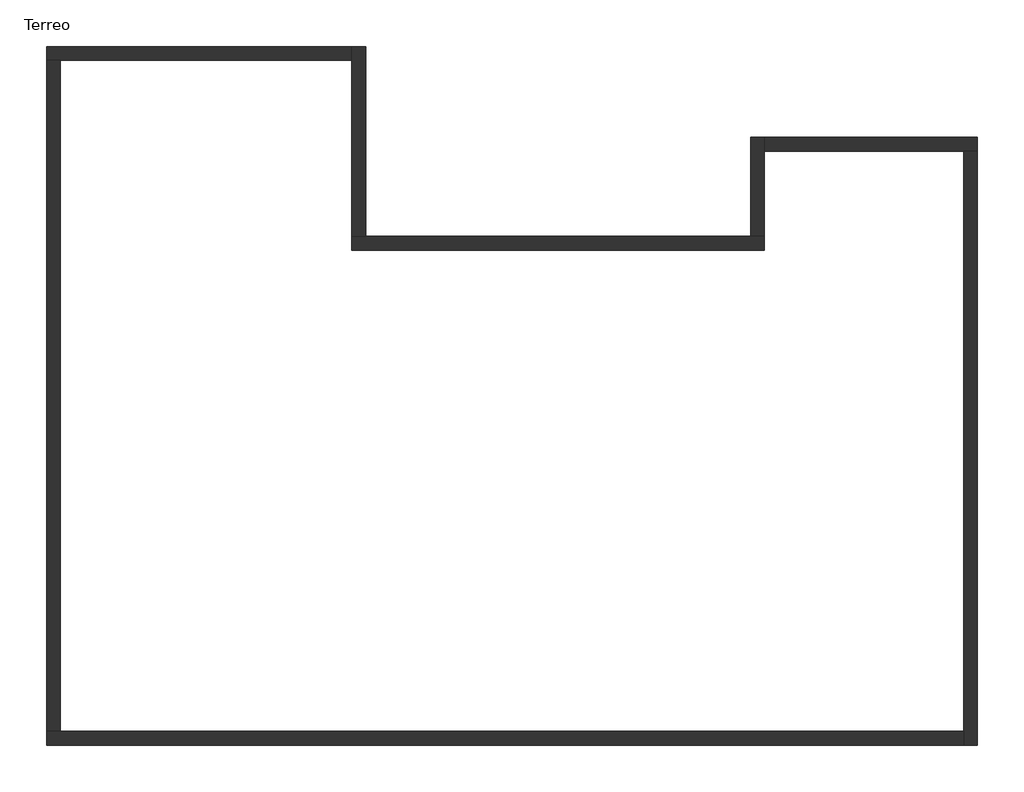
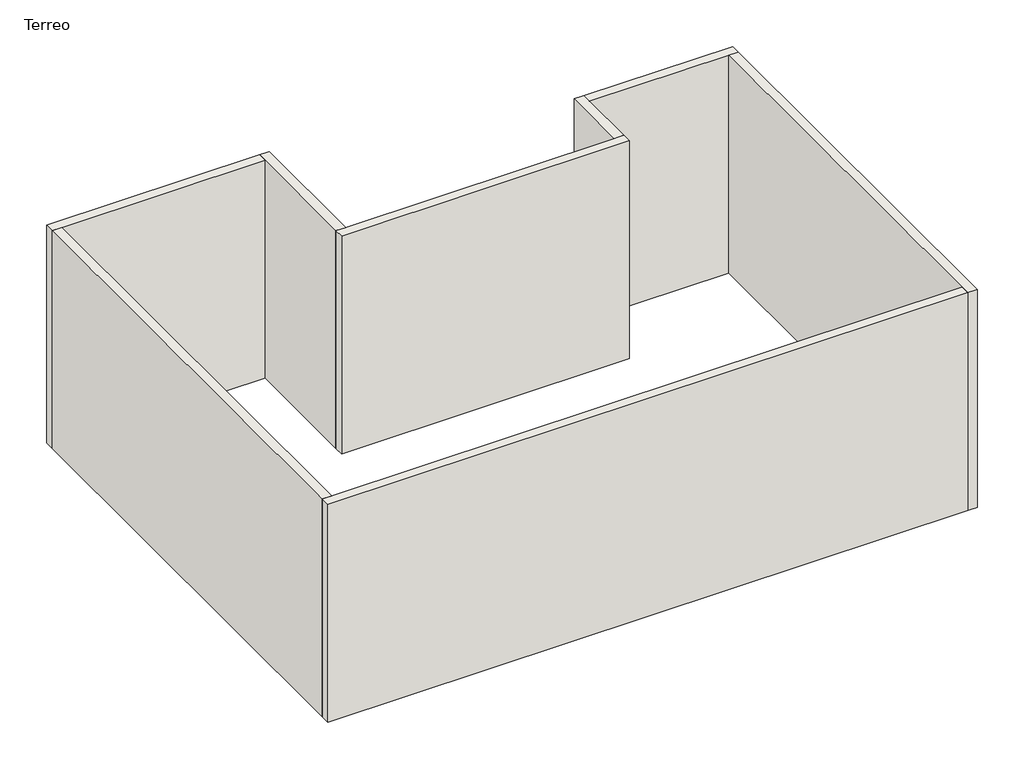
# One storey: 8 walls.
"""IFC4 building model written with IfcOpenShell, lengths in millimetres."""

import ifcopenshell
import ifcopenshell.guid

model = None  # the IFC model being written
_history = None  # IfcOwnerHistory: only IFC2X3 demands one
_inside = {}  # id of a spatial element -> (the spatial element, [elements in it])
_under = {}  # id of a project, library or spatial element -> (it, [spatial elements below it])
_declared = {}  # id of a project -> (the project, [libraries it declares])
_typed = {}  # id of a type object -> (the type object, [elements of that type])
_made_of = {}  # id of a material, layer set ... -> (it, [elements and type objects made of it])


def new_model(schema):
    """Start an empty IFC model of exactly this schema.

    Asked for "IFC4X3", IfcOpenShell would pick the latest addendum, in which some entities
    have other attributes; the version numbers below select the first issue.
    IFC2X3 requires an IfcOwnerHistory on every rooted entity: one is made here for all.
    """
    global model, _history
    if schema == "IFC4X3":
        model = ifcopenshell.file(schema_version=(4, 3, 0, 0))
    else:
        model = ifcopenshell.file(schema=schema)
    _inside.clear()
    _under.clear()
    _declared.clear()
    _typed.clear()
    _made_of.clear()
    _history = None
    if model.schema == "IFC2X3":
        org = make("IfcOrganization", Name="unknown")
        user = make(
            "IfcPersonAndOrganization",
            ThePerson=make("IfcPerson", FamilyName="unknown"),
            TheOrganization=org,
        )
        app = make(
            "IfcApplication",
            ApplicationDeveloper=org,
            Version="unknown",
            ApplicationFullName="unknown",
            ApplicationIdentifier="unknown",
        )
        _history = make(
            "IfcOwnerHistory",
            OwningUser=user,
            OwningApplication=app,
            ChangeAction="ADDED",
            CreationDate=0,
        )
    return model


def make(cls, **values):
    """One entity of the class cls with the attributes given. An attribute that is None is left unset."""
    return model.create_entity(
        cls, **{name: value for name, value in values.items() if value is not None}
    )


def rooted(cls, **values):
    """An entity with a GlobalId (a new one), such as an element, a storey or a relation."""
    return make(cls, GlobalId=ifcopenshell.guid.new(), OwnerHistory=_history, **values)


def si_unit(unit_type, name, prefix=None):
    """IfcSIUnit, for example si_unit("LENGTHUNIT", "METRE", prefix="MILLI")."""
    return make("IfcSIUnit", UnitType=unit_type, Prefix=prefix, Name=name)


def assignment(units):
    """IfcUnitAssignment: the units of a project."""
    return None if units is None else make("IfcUnitAssignment", Units=units)


def point(xyz):
    """IfcCartesianPoint."""
    return None if xyz is None else make("IfcCartesianPoint", Coordinates=xyz)


def direction(xyz):
    """IfcDirection."""
    return None if xyz is None else make("IfcDirection", DirectionRatios=xyz)


def frame(location, z_axis=None, x_axis=None):
    """IfcAxis2Placement3D, a coordinate frame: its origin and axes. An axis left out is left unset."""
    return make(
        "IfcAxis2Placement3D",
        Location=point(location),
        Axis=direction(z_axis),
        RefDirection=direction(x_axis),
    )


def origin():
    """The frame at (0, 0, 0) with its axes left unset."""
    return frame((0.0, 0.0, 0.0))


def origin_with_axes():
    """The frame at (0, 0, 0) with the z axis (0, 0, 1) and the x axis (1, 0, 0) written out."""
    return frame((0.0, 0.0, 0.0), z_axis=(0.0, 0.0, 1.0), x_axis=(1.0, 0.0, 0.0))


def place(relative_to, where):
    """IfcLocalPlacement: puts the frame where relative to a parent placement (None: the world)."""
    return make(
        "IfcLocalPlacement", PlacementRelTo=relative_to, RelativePlacement=where
    )


def context(
    kind, dimensions, precision=None, world=None, true_north=None, identifier=None
):
    """IfcGeometricRepresentationContext, for example the 3D "Model" context."""
    return make(
        "IfcGeometricRepresentationContext",
        ContextIdentifier=identifier,
        ContextType=kind,
        CoordinateSpaceDimension=dimensions,
        Precision=precision,
        WorldCoordinateSystem=world,
        TrueNorth=true_north,
    )


def project(units=None, contexts=None):
    """IfcProject with its units and contexts."""
    return rooted(
        "IfcProject",
        Name="project",
        RepresentationContexts=contexts,
        UnitsInContext=assignment(units),
    )


def spatial(cls, under=None, at=None, **own):
    """A site, building, storey or space (cls), placed at a placement, below another one or the project."""
    s = rooted(cls, ObjectPlacement=at, **own)
    if under is not None:
        _under.setdefault(under.id(), (under, []))[1].append(s)
    return s


def polyline(points):
    """IfcPolyline through the points."""
    return make("IfcPolyline", Points=[point(p) for p in points])


def outline(outer, holes=None, kind="AREA"):
    """IfcArbitraryClosedProfileDef: a profile drawn as a closed curve; with holes, ...WithVoids."""
    if holes is None:
        return make("IfcArbitraryClosedProfileDef", ProfileType=kind, OuterCurve=outer)
    return make(
        "IfcArbitraryProfileDefWithVoids",
        ProfileType=kind,
        OuterCurve=outer,
        InnerCurves=holes,
    )


def extrude(swept, where, along, depth):
    """IfcExtrudedAreaSolid: the profile swept, set in the frame where, extruded along a direction by depth."""
    return make(
        "IfcExtrudedAreaSolid",
        SweptArea=swept,
        Position=where,
        ExtrudedDirection=direction(along),
        Depth=depth,
    )


def faces_of(points, faces, orient=None, outer=None):
    """IfcFace entities. A face is a list of loops; a loop is a list of indices into points, from 0.

    orient and outer hold one flag for each loop. By default every Orientation is true, the
    first loop of a face is its IfcFaceOuterBound and the others are IfcFaceBound.
    """
    made = []
    for i, loops in enumerate(faces):
        bounds = []
        for j, loop in enumerate(loops):
            is_outer = j == 0 if outer is None else outer[i][j]
            bounds.append(
                make(
                    "IfcFaceOuterBound" if is_outer else "IfcFaceBound",
                    Bound=make("IfcPolyLoop", Polygon=[points[k] for k in loop]),
                    Orientation=True if orient is None else orient[i][j],
                )
            )
        made.append(make("IfcFace", Bounds=bounds))
    return made


def faceted_brep(points, faces, orient=None, outer=None, voids=None):
    """IfcFacetedBrep: a solid bounded by flat faces; with voids (closed shells), ...WithVoids."""
    shared = [point(p) for p in points]
    hull = make("IfcClosedShell", CfsFaces=faces_of(shared, faces, orient, outer))
    if voids is None:
        return make("IfcFacetedBrep", Outer=hull)
    return make(
        "IfcFacetedBrepWithVoids",
        Outer=hull,
        Voids=[
            make(cls, CfsFaces=faces_of(shared, fs, o, b)) for cls, fs, o, b in voids
        ],
    )


def shape(context_of_items, identifier, shape_type, items):
    """IfcShapeRepresentation: the items that make up one representation, for example the "Body"."""
    return make(
        "IfcShapeRepresentation",
        ContextOfItems=context_of_items,
        RepresentationIdentifier=identifier,
        RepresentationType=shape_type,
        Items=items,
    )


def made_of(thing, what):
    """Note that an element or type object is made of a material, layer set ...; save() writes the relation."""
    if what is not None:
        _made_of.setdefault(what.id(), (what, []))[1].append(thing)
    return thing


def element(
    cls,
    number,
    at=None,
    inside=None,
    cuts=None,
    type_object=None,
    material=None,
    context=None,
    identifier="Body",
    shape_type=None,
    held_by="IfcProductDefinitionShape",
    body=None,
    shapes=None,
    **own,
):
    """One element of the class cls, such as IfcWall. Its Tag is "e" and its number.

    at: its placement. inside: the storey or other place that contains it. cuts: it is an
    opening in that element (IfcRelVoidsElement). A single representation is given by context,
    identifier, shape_type and body (its items); several are given by shapes. held_by: the class
    of the entity that holds the representations. save() writes the other relations.
    """
    e = rooted(cls, Tag="e%d" % number, ObjectPlacement=at, **own)
    if body is not None:
        shapes = [shape(context, identifier, shape_type, body)]
    if shapes is not None:
        e.Representation = make(held_by, Representations=shapes)
    if inside is not None:
        _inside.setdefault(inside.id(), (inside, []))[1].append(e)
    if cuts is not None:
        rooted(
            "IfcRelVoidsElement", RelatingBuildingElement=cuts, RelatedOpeningElement=e
        )
    if type_object is not None:
        _typed.setdefault(type_object.id(), (type_object, []))[1].append(e)
    return made_of(e, material)


def aggregate(whole, parts):
    """IfcRelAggregates: a whole, such as a stair, and the parts it consists of."""
    return rooted("IfcRelAggregates", RelatingObject=whole, RelatedObjects=parts)


def save(model, path):
    """Write the relations noted so far, then the file.

    IfcRelAggregates (storeys below a building ...), IfcRelContainedInSpatialStructure (elements
    in a storey), IfcRelDefinesByType, IfcRelAssociatesMaterial and IfcRelDeclares: one each for
    every whole, place, type object, material and project.
    """
    for whole, parts in _under.values():
        aggregate(whole, parts)
    for where, things in _inside.values():
        rooted(
            "IfcRelContainedInSpatialStructure",
            RelatedElements=things,
            RelatingStructure=where,
        )
    for kind, things in _typed.values():
        rooted("IfcRelDefinesByType", RelatedObjects=things, RelatingType=kind)
    for what, things in _made_of.values():
        rooted("IfcRelAssociatesMaterial", RelatedObjects=things, RelatingMaterial=what)
    for by, libraries in _declared.values():
        rooted("IfcRelDeclares", RelatingContext=by, RelatedDefinitions=libraries)
    model.write(path)


model = new_model("IFC4")

# Units and contexts
model_context = context("Model", 3, world=origin())
ifc_project = project(units=[si_unit("LENGTHUNIT", "METRE", prefix="MILLI")], contexts=[model_context])

# Site, building, storey
site = spatial("IfcSite", under=ifc_project)
building = spatial("IfcBuilding", under=site)
storey = spatial("IfcBuildingStorey", under=building, Name="Terreo", Elevation=0.0)

# Walls
placement = place(None, origin())
element("IfcWall", 1, ObjectType="Parede Externa - Bloco de Concreto 19 - Pintura / Pintura", at=placement, inside=storey, context=model_context, shape_type="Brep", body=[
    faceted_brep([(-321.4408024, 4756.6494336, 0.0), (7178.5591976, 4756.6494336, 0.0), (7178.5591976, 4756.6494336, 6000.0), (-321.4408024, 4756.6494336, 6000.0), (-321.4408024, 5006.6494336, 0.0), (-321.4408024, 5006.6494336, 6000.0), (-71.4408024, 5006.6494336, 6000.0), (6928.5591976, 5006.6494336, 6000.0), (7178.5591976, 5006.6494336, 6000.0), (7178.5591976, 5006.6494336, 0.0), (6928.5591976, 5006.6494336, 0.0), (-71.4408024, 5006.6494336, 0.0)], [[[0, 1, 2, 3]], [[4, 5, 6, 7, 8, 9, 10, 11]], [[1, 0, 4, 11, 10, 9]], [[3, 2, 8, 7, 6, 5]], [[0, 3, 5, 4]], [[2, 1, 9, 8]]]),
])
element("IfcWall", 2, ObjectType="Parede Externa - Bloco de Concreto 19 - Pintura / Pintura", at=placement, inside=storey, context=model_context, shape_type="Brep", body=[
    faceted_brep([(10803.5591976, 6556.6494336, 0.0), (10803.5591976, -3993.3505664, 0.0), (10803.5591976, -4243.3505664, 0.0), (10803.5591976, -4243.3505664, 6000.0), (10803.5591976, -3993.3505664, 6000.0), (10803.5591976, 6556.6494336, 6000.0), (11053.5591976, 6556.6494336, 0.0), (11053.5591976, 6556.6494336, 6000.0), (11053.5591976, -4243.3505664, 6000.0), (11053.5591976, -4243.3505664, 0.0)], [[[0, 1, 2, 3, 4, 5]], [[6, 7, 8, 9]], [[2, 1, 0, 6, 9]], [[5, 4, 3, 8, 7]], [[0, 5, 7, 6]], [[3, 2, 9, 8]]]),
])
element("IfcWall", 3, ObjectType="Parede Externa - Bloco de Concreto 19 - Pintura / Pintura", at=placement, inside=storey, context=model_context, shape_type="Brep", body=[
    faceted_brep([(10803.5591976, -3993.3505664, 0.0), (-5621.4408024, -3993.3505664, 0.0), (-5871.4408024, -3993.3505664, 0.0), (-5871.4408024, -3993.3505664, 6000.0), (-5621.4408024, -3993.3505664, 6000.0), (10803.5591976, -3993.3505664, 6000.0), (10803.5591976, -4243.3505664, 0.0), (10803.5591976, -4243.3505664, 6000.0), (-5871.4408024, -4243.3505664, 6000.0), (-5871.4408024, -4243.3505664, 0.0)], [[[0, 1, 2, 3, 4, 5]], [[6, 7, 8, 9]], [[2, 1, 0, 6, 9]], [[5, 4, 3, 8, 7]], [[0, 5, 7, 6]], [[3, 2, 9, 8]]]),
])
element("IfcWall", 4, ObjectType="Parede Externa - Bloco de Concreto 19 - Pintura / Pintura", at=placement, inside=storey, context=model_context, shape_type="Brep", body=[
    faceted_brep([(-71.4408024, 5006.6494336, 0.0), (-71.4408024, 8456.6494336, 0.0), (-71.4408024, 8456.6494336, 6000.0), (-71.4408024, 5006.6494336, 6000.0), (-321.4408024, 5006.6494336, 0.0), (-321.4408024, 5006.6494336, 6000.0), (-321.4408024, 8206.6494336, 6000.0), (-321.4408024, 8456.6494336, 6000.0), (-321.4408024, 8456.6494336, 0.0), (-321.4408024, 8206.6494336, 0.0)], [[[0, 1, 2, 3]], [[4, 5, 6, 7, 8, 9]], [[1, 0, 4, 9, 8]], [[3, 2, 7, 6, 5]], [[0, 3, 5, 4]], [[2, 1, 8, 7]]]),
])
element("IfcWall", 5, ObjectType="Parede Externa - Bloco de Concreto 19 - Pintura / Pintura", at=placement, inside=storey, context=model_context, shape_type="Brep", body=[
    faceted_brep([(7178.5591976, 5006.6494336, 0.0), (7178.5591976, 6556.6494336, 0.0), (7178.5591976, 6806.6494336, 0.0), (7178.5591976, 6806.6494336, 6000.0), (7178.5591976, 6556.6494336, 6000.0), (7178.5591976, 5006.6494336, 6000.0), (6928.5591976, 5006.6494336, 0.0), (6928.5591976, 5006.6494336, 6000.0), (6928.5591976, 6806.6494336, 6000.0), (6928.5591976, 6806.6494336, 0.0)], [[[0, 1, 2, 3, 4, 5]], [[6, 7, 8, 9]], [[2, 1, 0, 6, 9]], [[5, 4, 3, 8, 7]], [[3, 2, 9, 8]], [[0, 5, 7, 6]]]),
])
element("IfcWall", 6, ObjectType="Parede Externa - Bloco de Concreto 19 - Pintura / Pintura", at=placement, inside=storey, context=model_context, shape_type="Brep", body=[
    faceted_brep([(7178.5591976, 6556.6494336, 0.0), (10803.5591976, 6556.6494336, 0.0), (11053.5591976, 6556.6494336, 0.0), (11053.5591976, 6556.6494336, 6000.0), (10803.5591976, 6556.6494336, 6000.0), (7178.5591976, 6556.6494336, 6000.0), (7178.5591976, 6806.6494336, 0.0), (7178.5591976, 6806.6494336, 6000.0), (11053.5591976, 6806.6494336, 6000.0), (11053.5591976, 6806.6494336, 0.0)], [[[0, 1, 2, 3, 4, 5]], [[6, 7, 8, 9]], [[2, 1, 0, 6, 9]], [[5, 4, 3, 8, 7]], [[0, 5, 7, 6]], [[3, 2, 9, 8]]]),
])
element("IfcWall", 7, ObjectType="Parede Externa - Bloco de Concreto 19 - Pintura / Pintura", at=placement, inside=storey, context=model_context, shape_type="Brep", body=[
    faceted_brep([(-5871.4408024, 8206.6494336, 0.0), (-5621.4408024, 8206.6494336, 0.0), (-321.4408024, 8206.6494336, 0.0), (-321.4408024, 8206.6494336, 6000.0), (-5621.4408024, 8206.6494336, 6000.0), (-5871.4408024, 8206.6494336, 6000.0), (-5871.4408024, 8456.6494336, 0.0), (-5871.4408024, 8456.6494336, 6000.0), (-321.4408024, 8456.6494336, 6000.0), (-321.4408024, 8456.6494336, 0.0)], [[[0, 1, 2, 3, 4, 5]], [[6, 7, 8, 9]], [[2, 1, 0, 6, 9]], [[5, 4, 3, 8, 7]], [[3, 2, 9, 8]], [[0, 5, 7, 6]]]),
])
element("IfcWall", 8, ObjectType="Parede Externa - Bloco de Concreto 19 - Pintura / Pintura", at=placement, inside=storey, context=model_context, shape_type="SweptSolid", body=[
    extrude(outline(polyline([(-5621.4408024, 8206.6494336), (-5621.4408024, -3993.3505664), (-5871.4408024, -3993.3505664), (-5871.4408024, 8206.6494336), (-5621.4408024, 8206.6494336)])), origin_with_axes(), (0.0, 0.0, 1.0), 6000.0),
])

save(model, "model.ifc")

# Revit data of these elements
# Project information
#   Data de emissão do projeto = "01/01/2010"
#   Status do projeto = "GDPProjetos.RVT"
#   Nome do cliente = "RAQUEL CANELLAS"
#   Endereço do projeto = "Av. Treze de Maio 13 sl.1414  |Centro | Rio de Janeiro"
#   Nome do projeto = "GDP - Gerenciamento e Desenvolvimento de Projetos"
#   Número do projeto = "100"
# Type "Parede Externa - Bloco de Concreto 19 - Pintura / Pintura"
#   Width = 0.25 m
#   Layers, outside or top first: 0.03 m "Emboço" (function 4); 0.19 m "Alvenaria" (function 1); 0.03 m "Emboço" (function 4)
# Elements 1, 2, 3, 4, 5, 6, 7 (IfcWall, "Parede Externa - Bloco de Concreto 19 - Pintura / Pintura")
#   Top Offset = 0.00 m
#   Base Offset = 0.00 m
#   wall height = 6.00 m
#   Phase Created = Construção Nova
#   Base Constraint = Terreo
#   Top Constraint = Cobertura
#   Materials on its faces: "Emboço", "Padrão - Parede"
# Element 8 (IfcWall, "Parede Externa - Bloco de Concreto 19 - Pintura / Pintura")
#   Top Offset = 0.00 m
#   Base Offset = 0.00 m
#   wall height = 6.00 m
#   Phase Created = Construção Nova
#   Base Constraint = Terreo
#   Top Constraint = Cobertura
#   Materials on its faces: "Padrão - Parede", "Emboço"
# Materials
#   "Emboço": class "Cimento", colour RGB 192 192 192, transparency 0, Cost = 0
#   "Alvenaria": colour RGB 249 249 249, transparency 0, Cost = 0
#   "Padrão - Parede": colour RGB 255 255 255, transparency 0, Cost = 0
